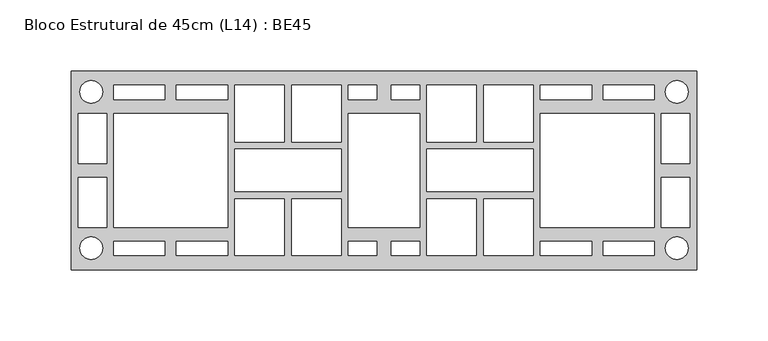
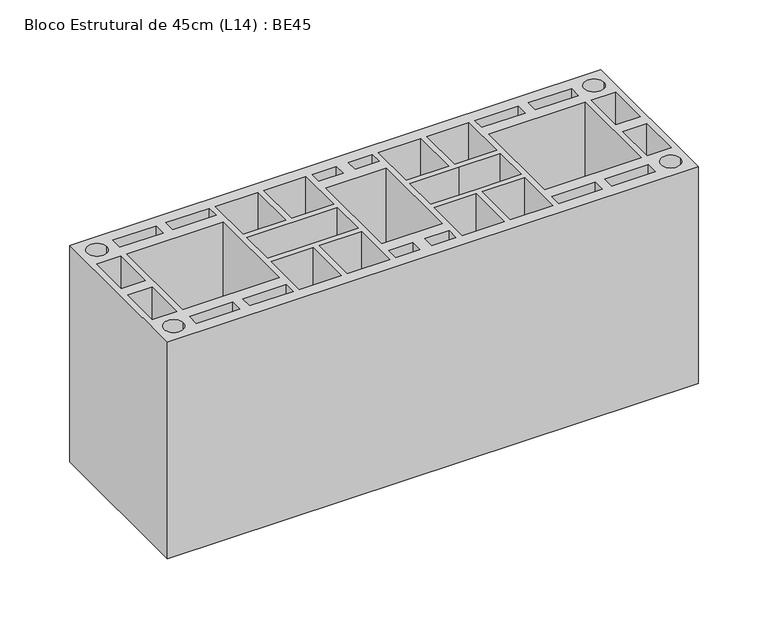
"""IFC4 building model written with IfcOpenShell, lengths in millimetres: proxy geometry, Bloco Estrutural de 45cm (L14) : BE45."""

from ifc_helpers import new_model, si_unit, point, frame_2d, origin, origin_with_axes, place, context, project, spatial, polyline, circle_curve, trimmed, segment, composite_curve, outline, extrude, source, transform, mapped, element, save


def bloco_estrutural_de_45cm_l14_be45_6e5ecc11(model_context):
    return source(origin(), model_context, "Body", "SweptSolid", [
        extrude(outline(polyline([(440.0, 0.0), (440.0, -140.0), (0.0, -140.0), (0.0, 0.0), (440.0, 0.0)]), holes=[composite_curve([segment(trimmed(circle_curve(frame_2d((14.1087523, -124.7509514)), 8.0), [point((6.1087523, -124.7509514))], [point((22.1087523, -124.7509514))], True, "CARTESIAN"), True, "CONTINUOUS"), segment(trimmed(circle_curve(frame_2d((14.1087523, -124.7509514)), 8.0), [point((22.1087523, -124.7509514))], [point((6.1087523, -124.7509514))], True, "CARTESIAN"), True, "CONTINUOUS")], self_intersect=False), composite_curve([segment(trimmed(circle_curve(frame_2d((14.1087523, -14.7509514)), 8.0), [point((6.1087523, -14.7509514))], [point((22.1087523, -14.7509514))], True, "CARTESIAN"), True, "CONTINUOUS"), segment(trimmed(circle_curve(frame_2d((14.1087523, -14.7509514)), 8.0), [point((22.1087523, -14.7509514))], [point((6.1087523, -14.7509514))], True, "CARTESIAN"), True, "CONTINUOUS")], self_intersect=False), polyline([(110.0, -110.0), (110.0, -30.0), (30.0, -30.0), (30.0, -110.0), (110.0, -110.0)]), polyline([(245.0, -110.0), (245.0, -30.0), (195.0, -30.0), (195.0, -110.0), (245.0, -110.0)]), polyline([(66.0, -130.0), (66.0, -120.0), (30.0, -120.0), (30.0, -130.0), (66.0, -130.0)]), polyline([(66.0, -20.0), (66.0, -10.0), (30.0, -10.0), (30.0, -20.0), (66.0, -20.0)]), polyline([(74.0, -130.0), (110.0, -130.0), (110.0, -120.0), (74.0, -120.0), (74.0, -130.0)]), polyline([(74.0, -20.0), (110.0, -20.0), (110.0, -10.0), (74.0, -10.0), (74.0, -20.0)]), composite_curve([segment(trimmed(circle_curve(frame_2d((425.8912477, -124.7509514)), 8.0), [point((433.8912477, -124.7509514))], [point((417.8912477, -124.7509514))], True, "CARTESIAN"), True, "CONTINUOUS"), segment(trimmed(circle_curve(frame_2d((425.8912477, -124.7509514)), 8.0), [point((417.8912477, -124.7509514))], [point((433.8912477, -124.7509514))], True, "CARTESIAN"), True, "CONTINUOUS")], self_intersect=False), composite_curve([segment(trimmed(circle_curve(frame_2d((425.8912477, -14.7509514)), 8.0), [point((433.8912477, -14.7509514))], [point((417.8912477, -14.7509514))], True, "CARTESIAN"), True, "CONTINUOUS"), segment(trimmed(circle_curve(frame_2d((425.8912477, -14.7509514)), 8.0), [point((417.8912477, -14.7509514))], [point((433.8912477, -14.7509514))], True, "CARTESIAN"), True, "CONTINUOUS")], self_intersect=False), polyline([(330.0, -110.0), (410.0, -110.0), (410.0, -30.0), (330.0, -30.0), (330.0, -110.0)]), polyline([(374.0, -130.0), (410.0, -130.0), (410.0, -120.0), (374.0, -120.0), (374.0, -130.0)]), polyline([(374.0, -20.0), (410.0, -20.0), (410.0, -10.0), (374.0, -10.0), (374.0, -20.0)]), polyline([(366.0, -130.0), (366.0, -120.0), (330.0, -120.0), (330.0, -130.0), (366.0, -130.0)]), polyline([(366.0, -20.0), (366.0, -10.0), (330.0, -10.0), (330.0, -20.0), (366.0, -20.0)]), polyline([(25.0, -110.0), (25.0, -75.0), (5.0, -75.0), (5.0, -110.0), (25.0, -110.0)]), polyline([(25.0, -30.0), (5.0, -30.0), (5.0, -65.0), (25.0, -65.0), (25.0, -30.0)]), polyline([(415.0, -110.0), (435.0, -110.0), (435.0, -75.0), (415.0, -75.0), (415.0, -110.0)]), polyline([(415.0, -30.0), (415.0, -65.0), (435.0, -65.0), (435.0, -30.0), (415.0, -30.0)]), polyline([(225.0, -20.0), (245.0, -20.0), (245.0, -10.0), (225.0, -10.0), (225.0, -20.0)]), polyline([(215.0, -20.0), (215.0, -10.0), (195.0, -10.0), (195.0, -20.0), (215.0, -20.0)]), polyline([(225.0, -120.0), (225.0, -130.0), (245.0, -130.0), (245.0, -120.0), (225.0, -120.0)]), polyline([(215.0, -120.0), (195.0, -120.0), (195.0, -130.0), (215.0, -130.0), (215.0, -120.0)]), polyline([(150.0, -130.0), (150.0, -90.0), (115.0, -90.0), (115.0, -130.0), (150.0, -130.0)]), polyline([(190.0, -130.0), (190.0, -90.0), (155.0, -90.0), (155.0, -130.0), (190.0, -130.0)]), polyline([(115.0, -85.0), (148.9828076, -85.0), (190.0, -85.0), (190.0, -55.0), (115.0, -55.0), (115.0, -85.0)]), polyline([(155.0, -50.0), (190.0, -50.0), (190.0, -10.0), (155.0, -10.0), (155.0, -50.0)]), polyline([(150.0, -10.0), (115.0, -10.0), (115.0, -50.0), (150.0, -50.0), (150.0, -10.0)]), polyline([(290.0, -130.0), (325.0, -130.0), (325.0, -90.0), (290.0, -90.0), (290.0, -130.0)]), polyline([(250.0, -130.0), (285.0, -130.0), (285.0, -90.0), (250.0, -90.0), (250.0, -130.0)]), polyline([(325.0, -85.0), (325.0, -55.0), (291.0171924, -55.0), (250.0, -55.0), (250.0, -85.0), (291.0171924, -85.0), (325.0, -85.0)]), polyline([(285.0, -50.0), (285.0, -10.0), (250.0, -10.0), (250.0, -50.0), (285.0, -50.0)]), polyline([(290.0, -10.0), (290.0, -50.0), (325.0, -50.0), (325.0, -10.0), (290.0, -10.0)])]), origin_with_axes(), (0.0, 0.0, 1.0), 190.0),
    ])


if __name__ == "__main__":
    model = new_model("IFC4")
    model_context = context("Model", 3, world=origin())
    ifc_project = project(units=[si_unit("LENGTHUNIT", "METRE", prefix="MILLI")], contexts=[model_context])
    site = spatial("IfcSite", under=ifc_project)
    building = spatial("IfcBuilding", under=site)
    placement = place(None, origin())
    bloco_estrutural_de_45cm_l14_be45_shape = bloco_estrutural_de_45cm_l14_be45_6e5ecc11(model_context)
    element("IfcBuildingElementProxy", 1, Name="Bloco Estrutural de 45cm (L14) : BE45", ObjectType="Bloco Estrutural de 45cm (L14) : BE45", at=placement, inside=building, context=model_context, shape_type="MappedRepresentation", body=[
        mapped(bloco_estrutural_de_45cm_l14_be45_shape, transform((0.0, 0.0, 0.0), x_axis=(1.0, 0.0, 0.0), y_axis=(0.0, 1.0, 0.0), z_axis=(0.0, 0.0, 1.0))),
    ])
    save(model, "model.ifc")

# Revit data of these elements
# Type "Bloco Estrutural de 45cm (L14) : BE45"
#   Material [instance default] = Blocos Cerâmicos
#   Default Elevation = 0
# Element 1 (IfcBuildingElementProxy, "Bloco Estrutural de 45cm (L14) : BE45")
#   Materials on its faces: "Blocos Cerâmicos"
# Materials
#   "Blocos Cerâmicos": class "Genérico", colour RGB 177 84 47, transparency 0, Cost = 0
